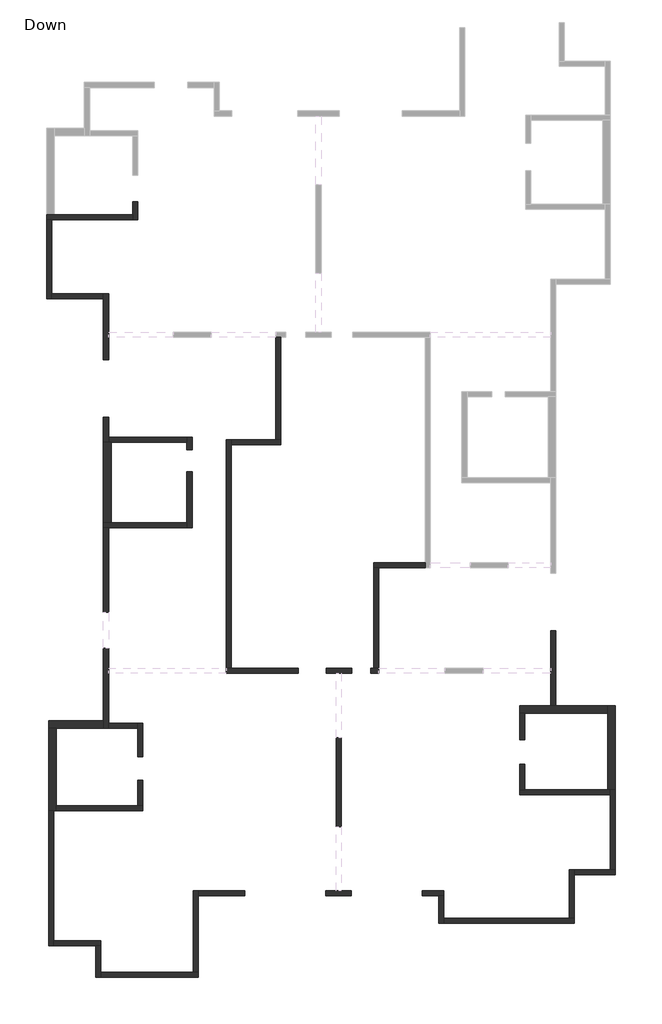
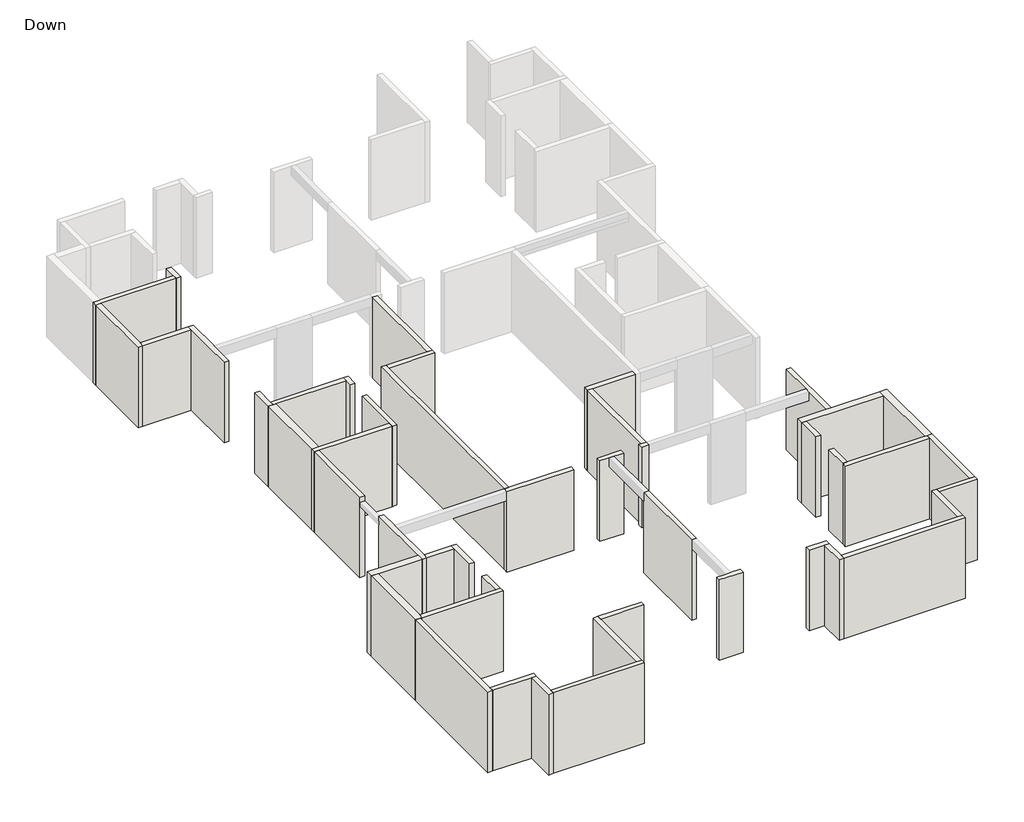
# One storey, part 1 of 2: 47 walls.
# Revit data of these elements (continued)
# Element 36 (IfcWall, "20") (continued)
#   Top Offset = 0 cm
#   Base Offset = 0 cm
#   wall height = 360 cm
#   SOFiSTiK_AMG_Scheduled = yes
#   SOFiSTiK_AMG_Adjusted = yes
#   Phase Created = New Construction
#   Base Constraint = Down
#   Top Constraint = Typical Floor
#   Materials on its faces: "Concrete"
# Element 37 (IfcWall, "20")
#   Comments = ""
#   Mark = "W71"
#   SOFiSTiK_EdgeZones = "W72"
#   SOFiSTiK_AMG_Comments = ""
#   Top Offset = 0 cm
#   Base Offset = 0 cm
#   wall height = 360 cm
#   SOFiSTiK_AMG_Scheduled = yes
#   SOFiSTiK_AMG_Adjusted = yes
#   Phase Created = New Construction
#   Base Constraint = Down
#   Top Constraint = Typical Floor
#   Materials on its faces: "Concrete"
# Element 38 (IfcWall, "20")
#   Comments = ""
#   Mark = "W76"
#   SOFiSTiK_EdgeZones = "W77"
#   SOFiSTiK_AMG_Comments = ""
#   Top Offset = 0 cm
#   Base Offset = 0 cm
#   wall height = 360 cm
#   SOFiSTiK_AMG_Scheduled = yes
#   SOFiSTiK_AMG_Adjusted = yes
#   Phase Created = New Construction
#   Base Constraint = Down
#   Top Constraint = Typical Floor
#   Materials on its faces: "Concrete"
# Element 39 (IfcWall, "20")
#   Comments = ""
#   Mark = "W77"
#   SOFiSTiK_EdgeZones = "W78"
#   SOFiSTiK_AMG_Comments = ""
#   Top Offset = 0 cm
#   Base Offset = 0 cm
#   wall height = 360 cm
#   SOFiSTiK_AMG_Scheduled = yes
#   SOFiSTiK_AMG_Adjusted = yes
#   Phase Created = New Construction
#   Base Constraint = Down
#   Top Constraint = Typical Floor
#   Materials on its faces: "Concrete"
# Element 40 (IfcWall, "20")
#   Comments = ""
#   Mark = "W78"
#   SOFiSTiK_EdgeZones = "W79"
#   SOFiSTiK_AMG_Comments = ""
#   Top Offset = 0 cm
#   Base Offset = 0 cm
#   wall height = 360 cm
#   SOFiSTiK_AMG_Scheduled = yes
#   SOFiSTiK_AMG_Adjusted = yes
#   Phase Created = New Construction
#   Base Constraint = Down
#   Top Constraint = Typical Floor
#   Materials on its faces: "Concrete"
# Element 41 (IfcWall, "20")
#   Comments = ""
#   Mark = "W79"
#   SOFiSTiK_EdgeZones = "W80"
#   SOFiSTiK_AMG_Comments = ""
#   Top Offset = 0 cm
#   Base Offset = 0 cm
#   wall height = 360 cm
#   SOFiSTiK_AMG_Scheduled = yes
#   SOFiSTiK_AMG_Adjusted = yes
#   Phase Created = New Construction
#   Base Constraint = Down
#   Top Constraint = Typical Floor
#   Materials on its faces: "Concrete"
# Element 42 (IfcWall, "20")
#   Comments = ""
#   Mark = "W82"
#   SOFiSTiK_EdgeZones = "W27"
#   SOFiSTiK_AMG_Comments = ""
#   Top Offset = 0 cm
#   Base Offset = 0 cm
#   wall height = 360 cm
#   SOFiSTiK_AMG_Scheduled = yes
#   SOFiSTiK_AMG_Adjusted = yes
#   Phase Created = New Construction
#   Base Constraint = Down
#   Top Constraint = Typical Floor
#   Materials on its faces: "Concrete"
# Element 43 (IfcWall, "30")
#   Comments = ""
#   Mark = "W3"
#   SOFiSTiK_EdgeZones = "W3"
#   SOFiSTiK_AMG_Comments = ""
#   Top Offset = 0 cm
#   Base Offset = 0 cm
#   wall height = 360 cm
#   SOFiSTiK_AMG_Scheduled = yes
#   SOFiSTiK_AMG_Adjusted = yes
#   Phase Created = New Construction
#   Base Constraint = Down
#   Top Constraint = Typical Floor
#   Materials on its faces: "Concrete"
# Element 44 (IfcWall, "30")
#   Comments = ""
#   Mark = "W4"
#   SOFiSTiK_EdgeZones = "W4"
#   SOFiSTiK_AMG_Comments = ""
#   Top Offset = 0 cm
#   Base Offset = 0 cm
#   wall height = 360 cm
#   SOFiSTiK_AMG_Scheduled = yes
#   SOFiSTiK_AMG_Adjusted = yes
#   Phase Created = New Construction
#   Base Constraint = Down
#   Top Constraint = Typical Floor
#   Materials on its faces: "Concrete"
# Element 45 (IfcWall, "30")
#   Comments = ""
#   Mark = "W5"
#   SOFiSTiK_EdgeZones = "W5"
#   SOFiSTiK_AMG_Comments = ""
#   Top Offset = 0 cm
#   Base Offset = 0 cm
#   wall height = 360 cm
#   SOFiSTiK_AMG_Scheduled = yes
#   SOFiSTiK_AMG_Adjusted = yes
#   Phase Created = New Construction
#   Base Constraint = Down
#   Top Constraint = Typical Floor
#   Materials on its faces: "Concrete"
# Element 46 (IfcWall, "30")
#   Comments = ""
#   Mark = "W6"
#   SOFiSTiK_EdgeZones = "W6"
#   SOFiSTiK_AMG_Comments = ""
#   Top Offset = 0 cm
#   Base Offset = 0 cm
#   wall height = 360 cm
#   SOFiSTiK_AMG_Scheduled = yes
#   SOFiSTiK_AMG_Adjusted = yes
#   Phase Created = New Construction
#   Base Constraint = Down
#   Top Constraint = Typical Floor
#   Materials on its faces: "Concrete"
# Element 47 (IfcWall, "30")
#   Comments = ""
#   Mark = "W7"
#   SOFiSTiK_EdgeZones = "W7"
#   SOFiSTiK_AMG_Comments = ""
#   Top Offset = 0 cm
#   Base Offset = 0 cm
#   wall height = 360 cm
#   SOFiSTiK_AMG_Scheduled = yes
#   SOFiSTiK_AMG_Adjusted = yes
#   Phase Created = New Construction
#   Base Constraint = Down
#   Top Constraint = Typical Floor
#   Materials on its faces: "Concrete"
# Materials
#   "Concrete": class "Concrete", colour RGB 192 192 192, transparency 0, Keynote = "01000", Description = "Cast-in-place concrete", Cost = 0
